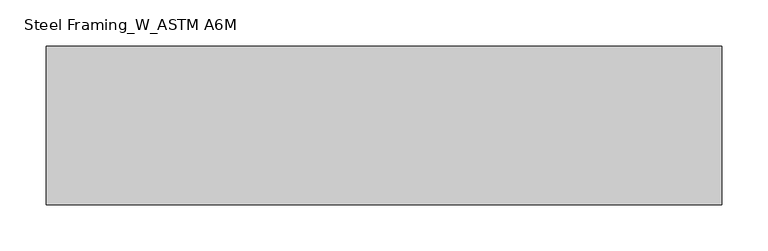
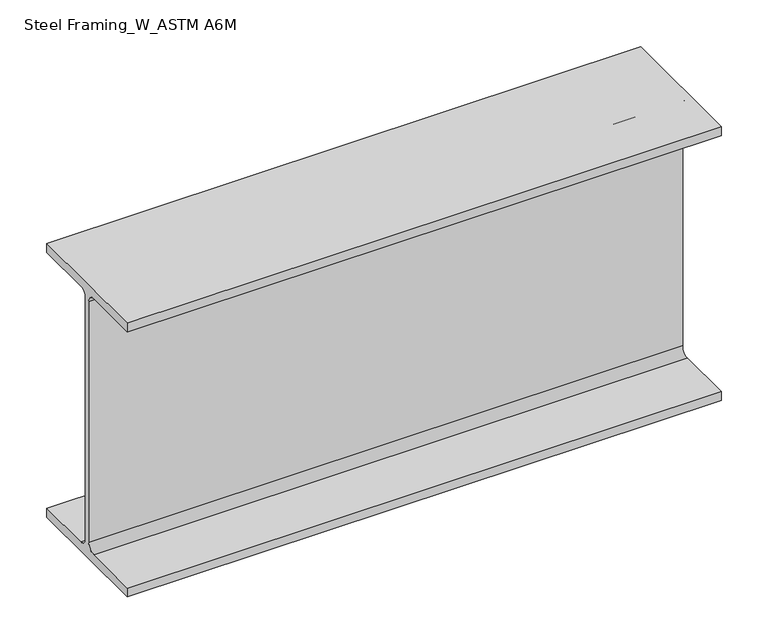
"""IFC4 building model written with IfcOpenShell, lengths in millimetres: beam geometry, Steel Framing_W_ASTM A6M : H_SB_AR_S02_W360x51_RG1."""

import ifcopenshell
import ifcopenshell.guid

model = None  # the IFC model being written
_history = None  # IfcOwnerHistory: only IFC2X3 demands one
_inside = {}  # id of a spatial element -> (the spatial element, [elements in it])
_under = {}  # id of a project, library or spatial element -> (it, [spatial elements below it])
_declared = {}  # id of a project -> (the project, [libraries it declares])
_typed = {}  # id of a type object -> (the type object, [elements of that type])
_made_of = {}  # id of a material, layer set ... -> (it, [elements and type objects made of it])


def new_model(schema):
    """Start an empty IFC model of exactly this schema.

    Asked for "IFC4X3", IfcOpenShell would pick the latest addendum, in which some entities
    have other attributes; the version numbers below select the first issue.
    IFC2X3 requires an IfcOwnerHistory on every rooted entity: one is made here for all.
    """
    global model, _history
    if schema == "IFC4X3":
        model = ifcopenshell.file(schema_version=(4, 3, 0, 0))
    else:
        model = ifcopenshell.file(schema=schema)
    _inside.clear()
    _under.clear()
    _declared.clear()
    _typed.clear()
    _made_of.clear()
    _history = None
    if model.schema == "IFC2X3":
        org = make("IfcOrganization", Name="unknown")
        user = make(
            "IfcPersonAndOrganization",
            ThePerson=make("IfcPerson", FamilyName="unknown"),
            TheOrganization=org,
        )
        app = make(
            "IfcApplication",
            ApplicationDeveloper=org,
            Version="unknown",
            ApplicationFullName="unknown",
            ApplicationIdentifier="unknown",
        )
        _history = make(
            "IfcOwnerHistory",
            OwningUser=user,
            OwningApplication=app,
            ChangeAction="ADDED",
            CreationDate=0,
        )
    return model


def make(cls, **values):
    """One entity of the class cls with the attributes given. An attribute that is None is left unset."""
    return model.create_entity(
        cls, **{name: value for name, value in values.items() if value is not None}
    )


def rooted(cls, **values):
    """An entity with a GlobalId (a new one), such as an element, a storey or a relation."""
    return make(cls, GlobalId=ifcopenshell.guid.new(), OwnerHistory=_history, **values)


def si_unit(unit_type, name, prefix=None):
    """IfcSIUnit, for example si_unit("LENGTHUNIT", "METRE", prefix="MILLI")."""
    return make("IfcSIUnit", UnitType=unit_type, Prefix=prefix, Name=name)


def assignment(units):
    """IfcUnitAssignment: the units of a project."""
    return None if units is None else make("IfcUnitAssignment", Units=units)


def point(xyz):
    """IfcCartesianPoint."""
    return None if xyz is None else make("IfcCartesianPoint", Coordinates=xyz)


def direction(xyz):
    """IfcDirection."""
    return None if xyz is None else make("IfcDirection", DirectionRatios=xyz)


def frame(location, z_axis=None, x_axis=None):
    """IfcAxis2Placement3D, a coordinate frame: its origin and axes. An axis left out is left unset."""
    return make(
        "IfcAxis2Placement3D",
        Location=point(location),
        Axis=direction(z_axis),
        RefDirection=direction(x_axis),
    )


def frame_2d(location, x_axis=None):
    """IfcAxis2Placement2D, a coordinate frame in the plane: its origin and x axis."""
    return make(
        "IfcAxis2Placement2D", Location=point(location), RefDirection=direction(x_axis)
    )


def origin():
    """The frame at (0, 0, 0) with its axes left unset."""
    return frame((0.0, 0.0, 0.0))


def place(relative_to, where):
    """IfcLocalPlacement: puts the frame where relative to a parent placement (None: the world)."""
    return make(
        "IfcLocalPlacement", PlacementRelTo=relative_to, RelativePlacement=where
    )


def context(
    kind, dimensions, precision=None, world=None, true_north=None, identifier=None
):
    """IfcGeometricRepresentationContext, for example the 3D "Model" context."""
    return make(
        "IfcGeometricRepresentationContext",
        ContextIdentifier=identifier,
        ContextType=kind,
        CoordinateSpaceDimension=dimensions,
        Precision=precision,
        WorldCoordinateSystem=world,
        TrueNorth=true_north,
    )


def project(units=None, contexts=None):
    """IfcProject with its units and contexts."""
    return rooted(
        "IfcProject",
        Name="project",
        RepresentationContexts=contexts,
        UnitsInContext=assignment(units),
    )


def spatial(cls, under=None, at=None, **own):
    """A site, building, storey or space (cls), placed at a placement, below another one or the project."""
    s = rooted(cls, ObjectPlacement=at, **own)
    if under is not None:
        _under.setdefault(under.id(), (under, []))[1].append(s)
    return s


def polyline(points):
    """IfcPolyline through the points."""
    return make("IfcPolyline", Points=[point(p) for p in points])


def circle_curve(where, radius):
    """IfcCircle in the frame where."""
    return make("IfcCircle", Position=where, Radius=radius)


def trimmed(basis, trim1, trim2, sense, master):
    """IfcTrimmedCurve: the piece of a basis curve between two trims."""
    return make(
        "IfcTrimmedCurve",
        BasisCurve=basis,
        Trim1=trim1,
        Trim2=trim2,
        SenseAgreement=sense,
        MasterRepresentation=master,
    )


def segment(curve, same_sense, transition):
    """IfcCompositeCurveSegment."""
    return make(
        "IfcCompositeCurveSegment",
        Transition=transition,
        SameSense=same_sense,
        ParentCurve=curve,
    )


def composite_curve(segments, self_intersect=None):
    """IfcCompositeCurve: segments joined end to end."""
    return make("IfcCompositeCurve", Segments=segments, SelfIntersect=self_intersect)


def outline(outer, holes=None, kind="AREA"):
    """IfcArbitraryClosedProfileDef: a profile drawn as a closed curve; with holes, ...WithVoids."""
    if holes is None:
        return make("IfcArbitraryClosedProfileDef", ProfileType=kind, OuterCurve=outer)
    return make(
        "IfcArbitraryProfileDefWithVoids",
        ProfileType=kind,
        OuterCurve=outer,
        InnerCurves=holes,
    )


def extrude(swept, where, along, depth):
    """IfcExtrudedAreaSolid: the profile swept, set in the frame where, extruded along a direction by depth."""
    return make(
        "IfcExtrudedAreaSolid",
        SweptArea=swept,
        Position=where,
        ExtrudedDirection=direction(along),
        Depth=depth,
    )


def shape(context_of_items, identifier, shape_type, items):
    """IfcShapeRepresentation: the items that make up one representation, for example the "Body"."""
    return make(
        "IfcShapeRepresentation",
        ContextOfItems=context_of_items,
        RepresentationIdentifier=identifier,
        RepresentationType=shape_type,
        Items=items,
    )


def source(mapping_origin, context_of_items, identifier, shape_type, items):
    """IfcRepresentationMap: a shape defined once, which mapped items show again and again."""
    return make(
        "IfcRepresentationMap",
        MappingOrigin=mapping_origin,
        MappedRepresentation=shape(context_of_items, identifier, shape_type, items),
    )


def transform(
    local_origin,
    x_axis=None,
    y_axis=None,
    z_axis=None,
    scale=None,
    scale2=None,
    scale3=None,
    uniform=True,
):
    """IfcCartesianTransformationOperator3D, or its non-uniform kind. x_axis, y_axis, z_axis: its Axis1, 2, 3."""
    if uniform:
        return make(
            "IfcCartesianTransformationOperator3D",
            Axis1=direction(x_axis),
            Axis2=direction(y_axis),
            LocalOrigin=point(local_origin),
            Scale=scale,
            Axis3=direction(z_axis),
        )
    return make(
        "IfcCartesianTransformationOperator3DnonUniform",
        Axis1=direction(x_axis),
        Axis2=direction(y_axis),
        LocalOrigin=point(local_origin),
        Scale=scale,
        Axis3=direction(z_axis),
        Scale2=scale2,
        Scale3=scale3,
    )


def mapped(mapping_source, mapping_target):
    """IfcMappedItem: shows the shape of a source again, moved by a transform."""
    return make(
        "IfcMappedItem", MappingSource=mapping_source, MappingTarget=mapping_target
    )


def made_of(thing, what):
    """Note that an element or type object is made of a material, layer set ...; save() writes the relation."""
    if what is not None:
        _made_of.setdefault(what.id(), (what, []))[1].append(thing)
    return thing


def element(
    cls,
    number,
    at=None,
    inside=None,
    cuts=None,
    type_object=None,
    material=None,
    context=None,
    identifier="Body",
    shape_type=None,
    held_by="IfcProductDefinitionShape",
    body=None,
    shapes=None,
    **own,
):
    """One element of the class cls, such as IfcWall. Its Tag is "e" and its number.

    at: its placement. inside: the storey or other place that contains it. cuts: it is an
    opening in that element (IfcRelVoidsElement). A single representation is given by context,
    identifier, shape_type and body (its items); several are given by shapes. held_by: the class
    of the entity that holds the representations. save() writes the other relations.
    """
    e = rooted(cls, Tag="e%d" % number, ObjectPlacement=at, **own)
    if body is not None:
        shapes = [shape(context, identifier, shape_type, body)]
    if shapes is not None:
        e.Representation = make(held_by, Representations=shapes)
    if inside is not None:
        _inside.setdefault(inside.id(), (inside, []))[1].append(e)
    if cuts is not None:
        rooted(
            "IfcRelVoidsElement", RelatingBuildingElement=cuts, RelatedOpeningElement=e
        )
    if type_object is not None:
        _typed.setdefault(type_object.id(), (type_object, []))[1].append(e)
    return made_of(e, material)


def aggregate(whole, parts):
    """IfcRelAggregates: a whole, such as a stair, and the parts it consists of."""
    return rooted("IfcRelAggregates", RelatingObject=whole, RelatedObjects=parts)


def save(model, path):
    """Write the relations noted so far, then the file.

    IfcRelAggregates (storeys below a building ...), IfcRelContainedInSpatialStructure (elements
    in a storey), IfcRelDefinesByType, IfcRelAssociatesMaterial and IfcRelDeclares: one each for
    every whole, place, type object, material and project.
    """
    for whole, parts in _under.values():
        aggregate(whole, parts)
    for where, things in _inside.values():
        rooted(
            "IfcRelContainedInSpatialStructure",
            RelatedElements=things,
            RelatingStructure=where,
        )
    for kind, things in _typed.values():
        rooted("IfcRelDefinesByType", RelatedObjects=things, RelatingType=kind)
    for what, things in _made_of.values():
        rooted("IfcRelAssociatesMaterial", RelatedObjects=things, RelatingMaterial=what)
    for by, libraries in _declared.values():
        rooted("IfcRelDeclares", RelatingContext=by, RelatedDefinitions=libraries)
    model.write(path)


def steel_framing_w_astm_a6m_720331e8(model_context):
    return source(origin(), model_context, "Body", "SweptSolid", [
        extrude(outline(composite_curve([segment(polyline([(85.5, -166.4), (85.5, -178.0), (-85.5, -178.0), (-85.5, -166.4), (-13.72, -166.4)]), True, "CONTINUOUS"), segment(trimmed(circle_curve(frame_2d((-13.72, -156.3)), 10.1), [point((-13.72, -166.4))], [point((-3.62, -156.3))], True, "CARTESIAN"), True, "CONTINUOUS"), segment(polyline([(-3.62, -156.3), (-3.62, 156.3)]), True, "CONTINUOUS"), segment(trimmed(circle_curve(frame_2d((-13.72, 156.3)), 10.1), [point((-3.62, 156.3))], [point((-13.72, 166.4))], True, "CARTESIAN"), True, "CONTINUOUS"), segment(polyline([(-13.72, 166.4), (-85.5, 166.4), (-85.5, 178.0), (85.5, 178.0), (85.5, 166.4), (13.72, 166.4)]), True, "CONTINUOUS"), segment(trimmed(circle_curve(frame_2d((13.72, 156.3)), 10.1), [point((13.72, 166.4))], [point((3.62, 156.3))], True, "CARTESIAN"), True, "CONTINUOUS"), segment(polyline([(3.62, 156.3), (3.62, -156.3)]), True, "CONTINUOUS"), segment(trimmed(circle_curve(frame_2d((13.72, -156.3)), 10.1), [point((3.62, -156.3))], [point((13.72, -166.4))], True, "CARTESIAN"), True, "CONTINUOUS"), segment(polyline([(13.72, -166.4), (85.5, -166.4)]), True, "CONTINUOUS")], self_intersect=False)), frame((-229.55, 0.0, 0.0), z_axis=(1.0, 0.0, 0.0), x_axis=(0.0, 1.0, 0.0)), (0.0, 0.0, 1.0), 729.4),
    ])


if __name__ == "__main__":
    model = new_model("IFC4")
    model_context = context("Model", 3, world=origin())
    ifc_project = project(units=[si_unit("LENGTHUNIT", "METRE", prefix="MILLI")], contexts=[model_context])
    site = spatial("IfcSite", under=ifc_project)
    building = spatial("IfcBuilding", under=site)
    placement = place(None, origin())
    steel_framing_w_astm_a6m_shape = steel_framing_w_astm_a6m_720331e8(model_context)
    element("IfcBeam", 1, ObjectType="Steel Framing_W_ASTM A6M : H_SB_AR_S02_W360x51_RG1", at=placement, inside=building, context=model_context, shape_type="MappedRepresentation", body=[
        mapped(steel_framing_w_astm_a6m_shape, transform((0.0, 0.0, 0.0), x_axis=(1.0, 0.0, 0.0), y_axis=(0.0, 1.0, 0.0), z_axis=(0.0, 0.0, 1.0))),
    ])
    save(model, "model.ifc")

# Revit data of these elements
# Type "Steel Framing_W_ASTM A6M : H_SB_AR_S02_W360x51_RG1"
#   Type Mark = "RG1"
#   Section Name Key = "W14x34"
#   Width = 17.1 cm
#   Web Thickness = 0.724 cm
#   Web Fillet = 1.01 cm
#   Warping Constant = 287000.0 cm⁶
#   Torsional Moment of Inertia = 23.70 cm⁴
#   Section Area = 64.5 cm²
#   Plastic Modulus weak axis = 174.0 cm³
#   Plastic Modulus strong axis = 895.0 cm³
#   Perimeter = 1.36 m²/m
#   Nominal Weight = 51.00 kgf/m
#   Moment of Inertia weak axis = 970.00 cm⁴
#   Moment of Inertia strong axis = 14200.00 cm⁴
#   Height = 35.6 cm
#   Flange Thickness = 1.16 cm
#   Elastic Modulus weak axis = 113.0 cm³
#   Elastic Modulus strong axis = 796.0 cm³
#   Centroid Vertical = 17.8 cm
#   Centroid Horizontal = 8.55 cm
#   Length [instance default] = 1500 mm
#   Structural Material [instance default] = Steel, 45-345
#   Bolt Spacing = 0
#   Assembly Code = ""
# Element 1 (IfcBeam, "Steel Framing_W_ASTM A6M : H_SB_AR_S02_W360x51_RG1")
#   Materials on its faces: "Steel, 45-345"
# Materials
#   "Steel, 45-345": class "Metal", colour RGB 189 187 185, transparency 0, Description = "Steel 345 MPa", Cost = 0
